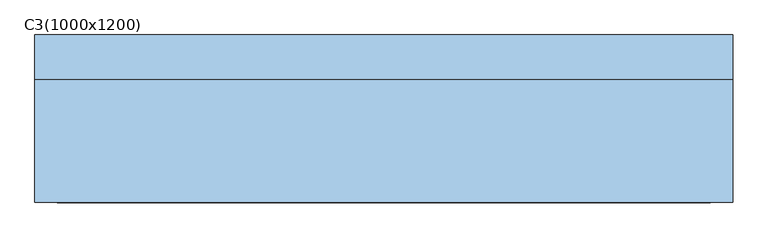
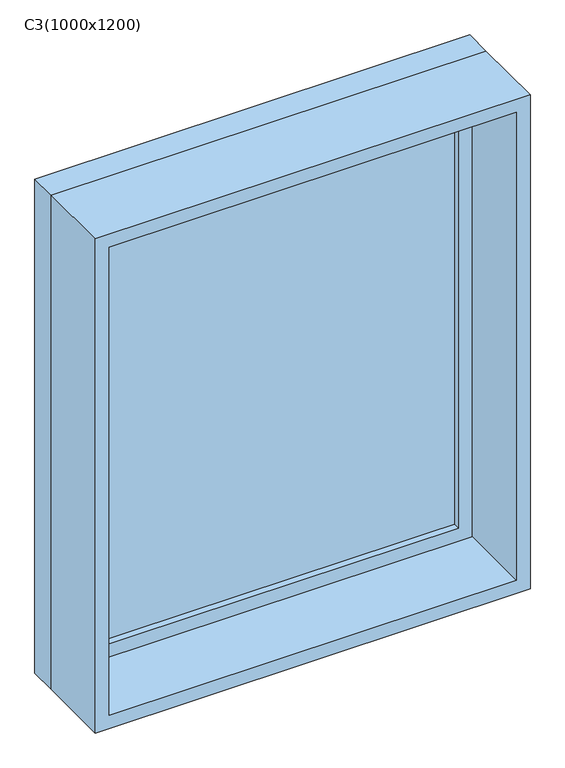
"""IFC4 building model written with IfcOpenShell, lengths in millimetres: window geometry, 固定窗 : C3(1000x1200)."""

from ifc_helpers import new_model, si_unit, frame, origin, place, context, project, spatial, polyline, outline, extrude, source, transform, mapped, element, save


def c3_1000x1200_4273239b(model_context):
    return source(origin(), model_context, "Body", "SweptSolid", [
        extrude(outline(polyline([(398.4, 71.425), (-474.6, 71.425), (-474.6, 84.125), (398.4, 84.125), (398.4, 71.425)])), frame((0.0, 0.0, 963.5), z_axis=(0.0, 0.0, 1.0), x_axis=(1.0, 0.0, 0.0)), (0.0, 0.0, 1.0), 1073.0),
        extrude(outline(polyline([(2080.95, -519.05), (919.05, -519.05), (919.05, 442.85), (2080.95, 442.85), (2080.95, -519.05)]), holes=[polyline([(2036.5, -474.6), (2036.5, 398.4), (963.5, 398.4), (963.5, -474.6), (2036.5, -474.6)])]), frame((0.0, 55.55, 0.0), z_axis=(0.0, 1.0, 0.0), x_axis=(0.0, 0.0, 1.0)), (0.0, 0.0, 1.0), 44.45),
        extrude(outline(polyline([(2100.0, -538.1), (900.0, -538.1), (900.0, 461.9), (2100.0, 461.9), (2100.0, -538.1)]), holes=[polyline([(2068.25, -506.35), (2068.25, 430.15), (931.75, 430.15), (931.75, -506.35), (2068.25, -506.35)])]), frame((0.0, -120.0, 0.0), z_axis=(0.0, 1.0, 0.0), x_axis=(0.0, 0.0, 1.0)), (0.0, 0.0, 1.0), 175.55),
        extrude(outline(polyline([(2100.0, 461.9), (2100.0, -538.1), (900.0, -538.1), (900.0, 461.9), (2100.0, 461.9)]), holes=[polyline([(2080.95, 442.85), (919.05, 442.85), (919.05, -519.05), (2080.95, -519.05), (2080.95, 442.85)])]), frame((0.0, 55.55, 0.0), z_axis=(0.0, 1.0, 0.0), x_axis=(0.0, 0.0, 1.0)), (0.0, 0.0, 1.0), 64.45),
    ])


if __name__ == "__main__":
    model = new_model("IFC4")
    model_context = context("Model", 3, world=origin())
    ifc_project = project(units=[si_unit("LENGTHUNIT", "METRE", prefix="MILLI")], contexts=[model_context])
    site = spatial("IfcSite", under=ifc_project)
    building = spatial("IfcBuilding", under=site)
    placement = place(None, origin())
    c3_1000x1200_shape = c3_1000x1200_4273239b(model_context)
    element("IfcWindow", 1, ObjectType="固定窗 : C3(1000x1200)", at=placement, inside=building, context=model_context, shape_type="MappedRepresentation", body=[
        mapped(c3_1000x1200_shape, transform((0.0, 0.0, 0.0), x_axis=(1.0, 0.0, 0.0), y_axis=(0.0, 1.0, 0.0), z_axis=(0.0, 0.0, 1.0))),
    ])
    save(model, "model.ifc")

# Revit data of these elements
# Type "固定窗 : C3(1000x1200)"
#   Type Mark = "C1516"
#   Construction Type Id = "SGL"
#   Analytic Construction = "大型单层玻璃窗"
#   Visual Light Transmittance = 0.9
#   Solar Heat Gain Coefficient = 0.86
#   Rough Width = 1000 mm
#   Rough Height = 1200 mm
#   Heat Transfer Coefficient (U) = 5.5617 W/(m²·K)
#   Height = 1200 mm
#   默认窗台高度 = 900 mm
#   Width = 1000 mm
#   窗嵌入 = 20 mm
#   高窗平面 [instance default] = no
#   通用窗平面 [instance default] = yes
#   玻璃 = none
#   框架材质 = none
#   Wall Closure = (empty or 0)
# Element 1 (IfcWindow, "固定窗 : C3(1000x1200)")
#   Materials on its faces: "玻璃"
# Materials
#   "玻璃": class "玻璃", colour RGB 0 128 192, transparency 0.9, Description = "钠钙玻璃", Cost = 0
